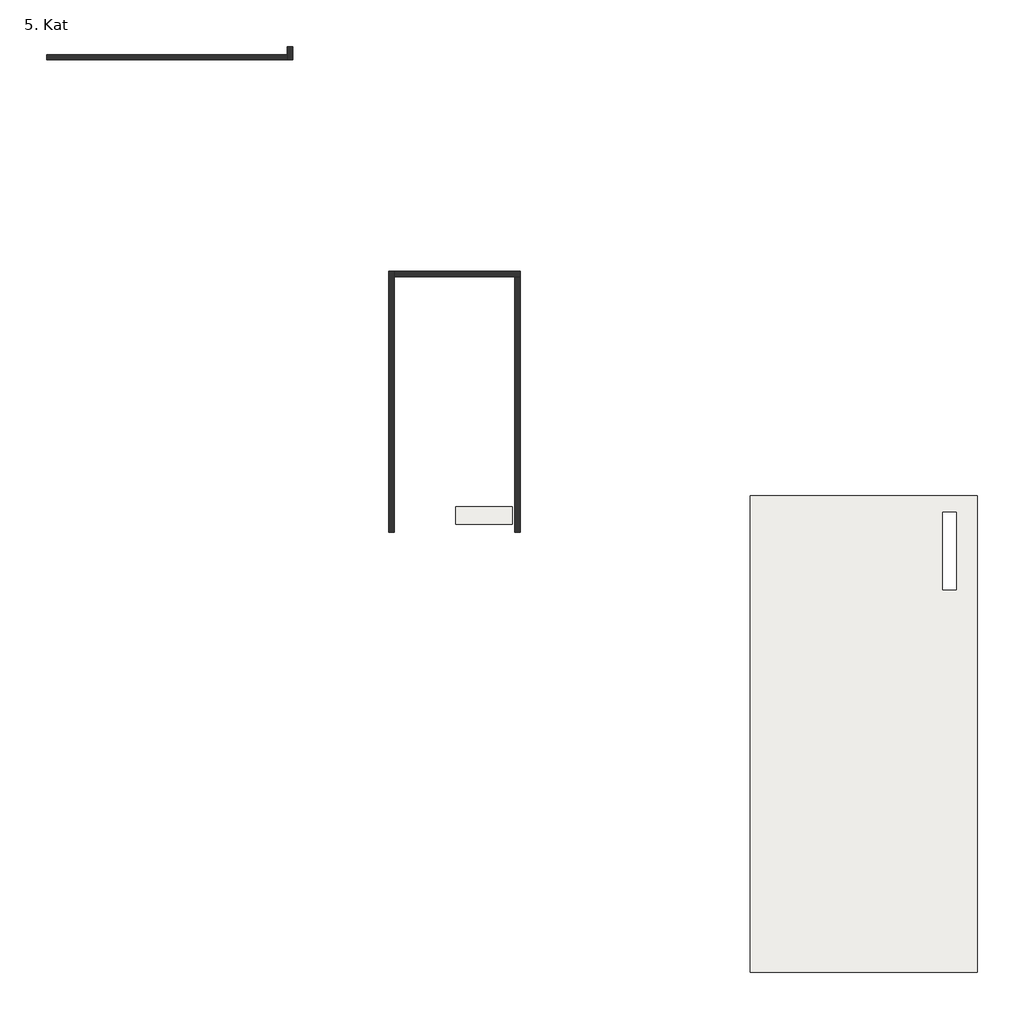
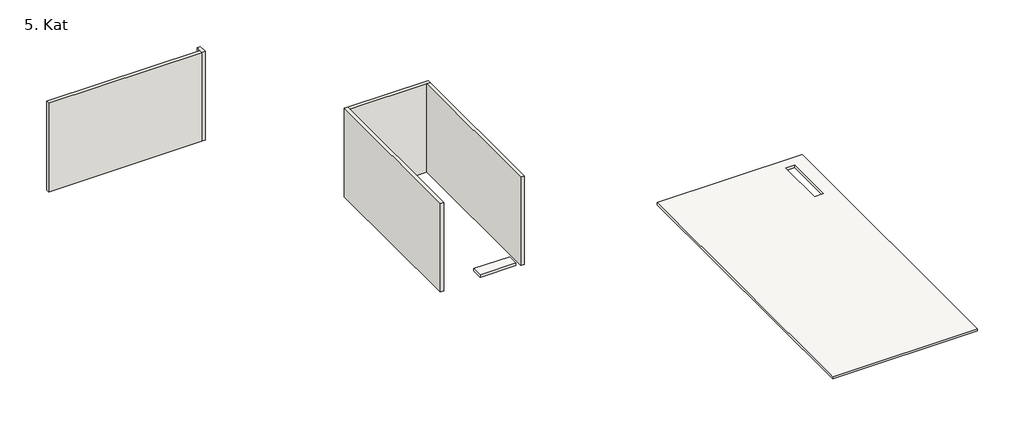
# One storey: 5 walls, 2 slabs.
"""IFC4 building model written with IfcOpenShell, lengths in millimetres."""

from ifc_helpers import new_model, si_unit, frame, origin, place, context, project, spatial, polyline, outline, extrude, faceted_brep, element, save

model = new_model("IFC4")

# Units and contexts
model_context = context("Model", 3, world=origin())
ifc_project = project(units=[si_unit("LENGTHUNIT", "METRE", prefix="MILLI")], contexts=[model_context])

# Site, building, storey
site = spatial("IfcSite", under=ifc_project)
building = spatial("IfcBuilding", under=site)
storey = spatial("IfcBuildingStorey", under=building, Name="5. Kat", Elevation=26500.0)

# Slabs
placement = place(None, origin())
element("IfcSlab", 1, ObjectType="Generic 150mm", at=placement, inside=storey, context=model_context, shape_type="SweptSolid", body=[
    extrude(outline(polyline([(34399.9997769, -399.9993776), (25900.0064017, -399.9993776), (25900.0064017, 17400.0011517), (34399.9997769, 17400.0011517), (34399.9997769, -399.9993776)]), holes=[polyline([(33099.999541, 13900.0015462), (33599.9997769, 13900.0015462), (33599.9997769, 16800.0015462), (33099.999541, 16800.0015462), (33099.999541, 13900.0015462)])]), frame((0.0, 0.0, 26350.0), z_axis=(0.0, 0.0, 1.0), x_axis=(1.0, 0.0, 0.0)), (0.0, 0.0, 1.0), 150.0),
])
element("IfcSlab", 2, ObjectType="Generic 150mm", at=placement, inside=storey, context=model_context, shape_type="SweptSolid", body=[
    extrude(outline(polyline([(14900.0010317, 16350.0011567), (14900.0010317, 17000.0011628), (17000.0064017, 17000.0011628), (17000.0064017, 16350.0011567), (14900.0010317, 16350.0011567)])), frame((0.0, 0.0, 26350.0), z_axis=(0.0, 0.0, 1.0), x_axis=(1.0, 0.0, 0.0)), (0.0, 0.0, 1.0), 150.0),
])

# Walls
element("IfcWall", 3, ObjectType="Generic - 200mm", at=placement, inside=storey, context=model_context, shape_type="SweptSolid", body=[
    extrude(outline(polyline([(8599.9995273, 33700.0009279), (-400.0005319, 33700.0009279), (-400.0005319, 33900.0009279), (8599.9995273, 33900.0009279), (8599.9995273, 33700.0009279)])), frame((0.0, 0.0, 26500.0), z_axis=(0.0, 0.0, 1.0), x_axis=(1.0, 0.0, 0.0)), (0.0, 0.0, 1.0), 5500.0),
])
element("IfcWall", 4, ObjectType="Generic - 200mm", at=placement, inside=storey, context=model_context, shape_type="Brep", body=[
    faceted_brep([(8799.9995273, 33700.0009279, 26500.0), (8799.9995273, 34200.0009279, 26500.0), (8799.9995273, 34200.0009279, 32000.0), (8799.9995273, 33700.0009279, 32000.0), (8599.9995273, 33700.0009279, 26500.0), (8599.9995273, 33700.0009279, 32000.0), (8599.9995273, 33900.0009279, 32000.0), (8599.9995273, 34200.0009279, 32000.0), (8599.9995273, 34200.0009279, 26500.0), (8599.9995273, 33900.0009279, 26500.0)], [[[0, 1, 2, 3]], [[4, 5, 6, 7, 8, 9]], [[1, 0, 4, 9, 8]], [[2, 1, 8, 7]], [[3, 2, 7, 6, 5]], [[0, 3, 5, 4]]]),
])
element("IfcWall", 5, ObjectType="Generic - 200mm", at=placement, inside=storey, context=model_context, shape_type="Brep", body=[
    faceted_brep([(12600.0064017, 16050.0009312, 26500.0), (12600.0064017, 25600.0006224, 26500.0), (12600.0064017, 25800.0006224, 26500.0), (12600.0064017, 25800.0006224, 32000.0), (12600.0064017, 25600.0006224, 32000.0), (12600.0064017, 16050.0009312, 32000.0), (12400.0064017, 16050.0009312, 26500.0), (12400.0064017, 16050.0009312, 32000.0), (12400.0064017, 25800.0006224, 32000.0), (12400.0064017, 25800.0006224, 26500.0)], [[[0, 1, 2, 3, 4, 5]], [[6, 7, 8, 9]], [[2, 1, 0, 6, 9]], [[5, 4, 3, 8, 7]], [[0, 5, 7, 6]], [[3, 2, 9, 8]]]),
])
element("IfcWall", 6, ObjectType="Generic - 200mm", at=placement, inside=storey, context=model_context, shape_type="Brep", body=[
    faceted_brep([(12600.0064017, 25600.0006224, 26500.0), (17100.0064017, 25600.0006224, 26500.0), (17300.0064017, 25600.0006224, 26500.0), (17300.0064017, 25600.0006224, 32000.0), (17100.0064017, 25600.0006224, 32000.0), (12600.0064017, 25600.0006224, 32000.0), (12600.0064017, 25800.0006224, 26500.0), (12600.0064017, 25800.0006224, 32000.0), (17300.0064017, 25800.0006224, 32000.0), (17300.0064017, 25800.0006224, 26500.0)], [[[0, 1, 2, 3, 4, 5]], [[6, 7, 8, 9]], [[2, 1, 0, 6, 9]], [[5, 4, 3, 8, 7]], [[3, 2, 9, 8]], [[0, 5, 7, 6]]]),
])
element("IfcWall", 7, ObjectType="Generic - 200mm", at=placement, inside=storey, context=model_context, shape_type="SweptSolid", body=[
    extrude(outline(polyline([(17100.0064017, 16050.0009312), (17100.0064017, 25600.0006224), (17300.0064017, 25600.0006224), (17300.0064017, 16050.0009312), (17100.0064017, 16050.0009312)])), frame((0.0, 0.0, 26500.0), z_axis=(0.0, 0.0, 1.0), x_axis=(1.0, 0.0, 0.0)), (0.0, 0.0, 1.0), 5500.0),
])

save(model, "model.ifc")

# Revit data of these elements
# Project information
#   Project Issue Date = "Issue Date"
#   Project Status = "Project Status"
#   Client Name = "Owner"
#   Project Address = "Enter address here"
#   Project Name = "Project Name"
#   Project Number = "0001"
# Grids (mm)
#   "1": line (0, 38461.009) -> (0, -4713.478)
#   "2": line (8500, 38461.009) -> (8500, -4713.478)
#   "3": line (12500, 38461.009) -> (12500, -4713.478)
#   "4": line (17000, 38461.009) -> (17000, -4713.478)
#   "5": line (25500, 38461.009) -> (25500, -4713.478)
#   "6": line (34000, 38461.009) -> (34000, -4713.478)
#   "A": line (-3152.065, 0.001) -> (40299.23, 0.001)
#   "B": line (-3152.065, 8500.001) -> (40299.23, 8500.001)
#   "C": line (-3152.065, 12500.001) -> (40299.23, 12500.001)
#   "D": line (-3152.065, 17000.001) -> (40299.23, 17000.001)
#   "E": line (-3152.065, 25500.001) -> (40299.23, 25500.001)
#   "F": line (-3152.065, 26450.001) -> (40299.23, 26450.001)
#   "G": line (-3152.065, 34000) -> (40299.23, 34000)
#   "H": line (0, 38461.009) -> (0, -4713.478)
#   "I": line (8500, 38461.009) -> (8500, -4713.478)
#   "J": line (12500, 38461.009) -> (12500, -4713.478)
#   "K": line (17000, 38461.009) -> (17000, -4713.478)
#   "L": line (25500, 38461.009) -> (25500, -4713.478)
#   "M": line (34000, 38461.009) -> (34000, -4713.478)
#   "N": line (-3152.065, 0.001) -> (40299.23, 0.001)
#   "O": line (-3152.065, 8500.001) -> (40299.23, 8500.001)
#   "P": line (-3152.065, 12500.001) -> (40299.23, 12500.001)
#   "Q": line (-3152.065, 17000.001) -> (40299.23, 17000.001)
#   "R": line (-3152.065, 25500.001) -> (40299.23, 25500.001)
#   "S": line (-3152.065, 26450.001) -> (40299.23, 26450.001)
#   "T": line (-3152.065, 34000) -> (40299.23, 34000)
# Type "Generic 150mm"
#   Function = 0
#   Layers, outside or top first: 15.00 cm no material (function 1)
# Type "Generic - 200mm"
#   Layers, outside or top first: 20.00 cm no material (function 1)
# Elements 1, 2 (IfcSlab, "Generic 150mm")
#   Height Offset From Level = 0.00 cm
#   Phase Created = New Construction
#   Materials on its faces: "Default Floor"
# Elements 3, 4, 5, 6, 7 (IfcWall, "Generic - 200mm")
#   Top Offset = 0.00 cm
#   Base Offset = 0.00 cm
#   Unconnected Height = 550.00 cm
#   wall height = 550.00 cm
#   Phase Created = New Construction
#   Base Constraint = 5. Kat
#   Top Constraint = 6. Kat
#   Materials on its faces: "Default Wall"
# Materials
#   "Default Floor": class "Miscellaneous", colour RGB 127 127 127, transparency 0, Cost = 0
#   "Default Wall": class "Miscellaneous", colour RGB 129 123 132, transparency 0, Cost = 0
